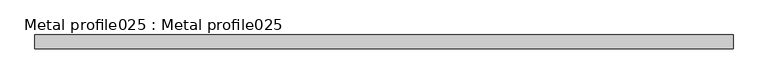
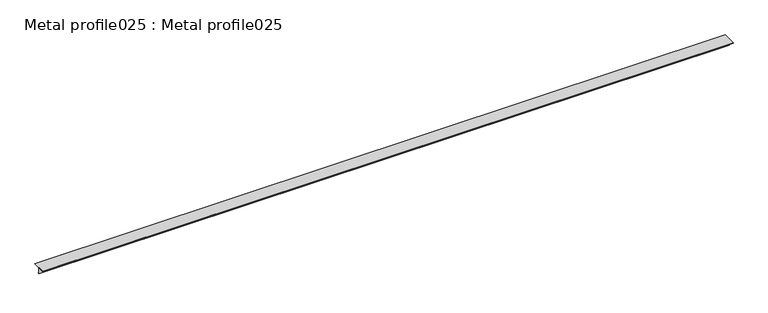
"""IFC4 building model written with IfcOpenShell, lengths in millimetres: proxy geometry, Metal profile025 : Metal profile025."""

from ifc_helpers import new_model, si_unit, frame, origin, place, context, project, spatial, polyline, outline, extrude, source, transform, mapped, element, save


def metal_profile025_metal_profile025_a14f86be(model_context):
    return source(origin(), model_context, "Body", "SweptSolid", [
        extrude(outline(polyline([(9776.5554633, 39551.5366067), (9780.0352633, 39551.5366067), (9780.0352633, 39550.2666067), (9775.2854633, 39550.2666067), (9775.2854633, 39568.5005547), (9756.2354633, 39568.5005547), (9756.2354633, 39569.7705547), (9795.6054633, 39569.7705547), (9795.6054633, 39568.5005547), (9776.5554633, 39568.5005547), (9776.5554633, 39551.5366067)])), frame((3694.2883192, 0.0, 0.0), z_axis=(1.0, 0.0, 0.0), x_axis=(0.0, 1.0, 0.0)), (0.0, 0.0, 1.0), 2000.0),
    ])


if __name__ == "__main__":
    model = new_model("IFC4")
    model_context = context("Model", 3, world=origin())
    ifc_project = project(units=[si_unit("LENGTHUNIT", "METRE", prefix="MILLI")], contexts=[model_context])
    site = spatial("IfcSite", under=ifc_project)
    building = spatial("IfcBuilding", under=site)
    placement = place(None, origin())
    metal_profile025_metal_profile025_shape = metal_profile025_metal_profile025_a14f86be(model_context)
    element("IfcBuildingElementProxy", 1, Name="Metal profile025 : Metal profile025", ObjectType="Metal profile025 : Metal profile025", at=placement, inside=building, context=model_context, shape_type="MappedRepresentation", body=[
        mapped(metal_profile025_metal_profile025_shape, transform((0.0, 0.0, 0.0), x_axis=(1.0, 0.0, 0.0), y_axis=(0.0, 1.0, 0.0), z_axis=(0.0, 0.0, 1.0))),
    ])
    save(model, "model.ifc")

# Revit data of these elements
# Type "Metal profile025 : Metal profile025"
#   NameOverride = "Metal profile025"
# Element 1 (IfcBuildingElementProxy, "Metal profile025 : Metal profile025")
#   Materials on its faces: "16 GA. COPPER VENTED T REVEAL BEAD"
# Materials
#   "16 GA. COPPER VENTED T REVEAL BEAD": class "Unassigned", colour RGB 255 227 10, transparency 0
